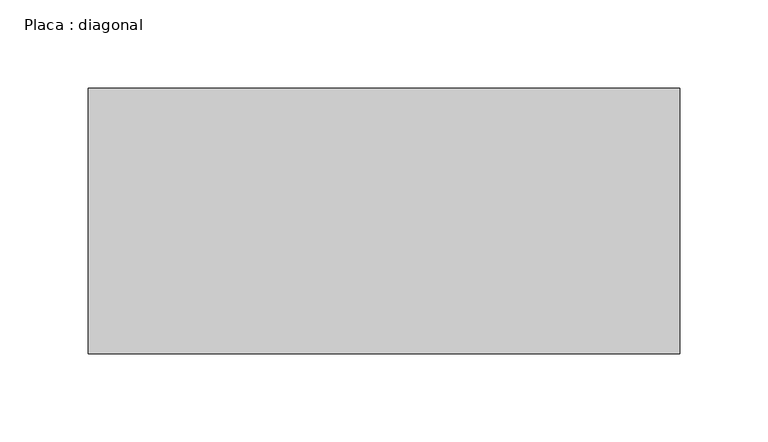
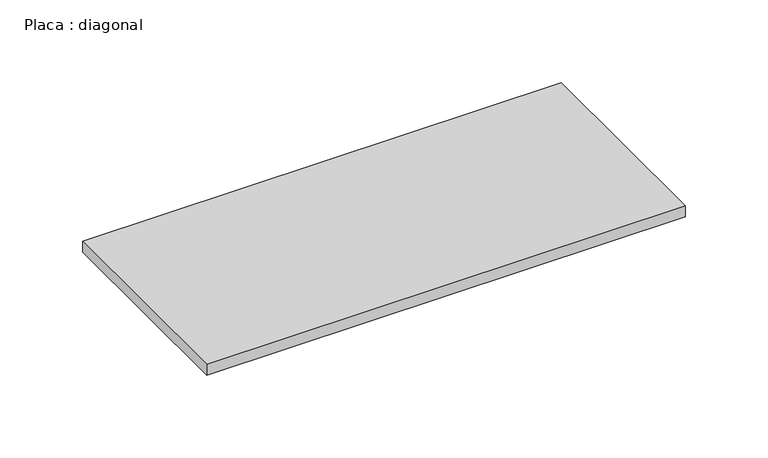
"""IFC4 building model written with IfcOpenShell, lengths in millimetres: beam geometry, Placa : diagonal."""

import ifcopenshell
import ifcopenshell.guid

model = None  # the IFC model being written
_history = None  # IfcOwnerHistory: only IFC2X3 demands one
_inside = {}  # id of a spatial element -> (the spatial element, [elements in it])
_under = {}  # id of a project, library or spatial element -> (it, [spatial elements below it])
_declared = {}  # id of a project -> (the project, [libraries it declares])
_typed = {}  # id of a type object -> (the type object, [elements of that type])
_made_of = {}  # id of a material, layer set ... -> (it, [elements and type objects made of it])


def new_model(schema):
    """Start an empty IFC model of exactly this schema.

    Asked for "IFC4X3", IfcOpenShell would pick the latest addendum, in which some entities
    have other attributes; the version numbers below select the first issue.
    IFC2X3 requires an IfcOwnerHistory on every rooted entity: one is made here for all.
    """
    global model, _history
    if schema == "IFC4X3":
        model = ifcopenshell.file(schema_version=(4, 3, 0, 0))
    else:
        model = ifcopenshell.file(schema=schema)
    _inside.clear()
    _under.clear()
    _declared.clear()
    _typed.clear()
    _made_of.clear()
    _history = None
    if model.schema == "IFC2X3":
        org = make("IfcOrganization", Name="unknown")
        user = make(
            "IfcPersonAndOrganization",
            ThePerson=make("IfcPerson", FamilyName="unknown"),
            TheOrganization=org,
        )
        app = make(
            "IfcApplication",
            ApplicationDeveloper=org,
            Version="unknown",
            ApplicationFullName="unknown",
            ApplicationIdentifier="unknown",
        )
        _history = make(
            "IfcOwnerHistory",
            OwningUser=user,
            OwningApplication=app,
            ChangeAction="ADDED",
            CreationDate=0,
        )
    return model


def make(cls, **values):
    """One entity of the class cls with the attributes given. An attribute that is None is left unset."""
    return model.create_entity(
        cls, **{name: value for name, value in values.items() if value is not None}
    )


def rooted(cls, **values):
    """An entity with a GlobalId (a new one), such as an element, a storey or a relation."""
    return make(cls, GlobalId=ifcopenshell.guid.new(), OwnerHistory=_history, **values)


def si_unit(unit_type, name, prefix=None):
    """IfcSIUnit, for example si_unit("LENGTHUNIT", "METRE", prefix="MILLI")."""
    return make("IfcSIUnit", UnitType=unit_type, Prefix=prefix, Name=name)


def assignment(units):
    """IfcUnitAssignment: the units of a project."""
    return None if units is None else make("IfcUnitAssignment", Units=units)


def point(xyz):
    """IfcCartesianPoint."""
    return None if xyz is None else make("IfcCartesianPoint", Coordinates=xyz)


def direction(xyz):
    """IfcDirection."""
    return None if xyz is None else make("IfcDirection", DirectionRatios=xyz)


def frame(location, z_axis=None, x_axis=None):
    """IfcAxis2Placement3D, a coordinate frame: its origin and axes. An axis left out is left unset."""
    return make(
        "IfcAxis2Placement3D",
        Location=point(location),
        Axis=direction(z_axis),
        RefDirection=direction(x_axis),
    )


def origin():
    """The frame at (0, 0, 0) with its axes left unset."""
    return frame((0.0, 0.0, 0.0))


def place(relative_to, where):
    """IfcLocalPlacement: puts the frame where relative to a parent placement (None: the world)."""
    return make(
        "IfcLocalPlacement", PlacementRelTo=relative_to, RelativePlacement=where
    )


def context(
    kind, dimensions, precision=None, world=None, true_north=None, identifier=None
):
    """IfcGeometricRepresentationContext, for example the 3D "Model" context."""
    return make(
        "IfcGeometricRepresentationContext",
        ContextIdentifier=identifier,
        ContextType=kind,
        CoordinateSpaceDimension=dimensions,
        Precision=precision,
        WorldCoordinateSystem=world,
        TrueNorth=true_north,
    )


def project(units=None, contexts=None):
    """IfcProject with its units and contexts."""
    return rooted(
        "IfcProject",
        Name="project",
        RepresentationContexts=contexts,
        UnitsInContext=assignment(units),
    )


def spatial(cls, under=None, at=None, **own):
    """A site, building, storey or space (cls), placed at a placement, below another one or the project."""
    s = rooted(cls, ObjectPlacement=at, **own)
    if under is not None:
        _under.setdefault(under.id(), (under, []))[1].append(s)
    return s


def polyline(points):
    """IfcPolyline through the points."""
    return make("IfcPolyline", Points=[point(p) for p in points])


def outline(outer, holes=None, kind="AREA"):
    """IfcArbitraryClosedProfileDef: a profile drawn as a closed curve; with holes, ...WithVoids."""
    if holes is None:
        return make("IfcArbitraryClosedProfileDef", ProfileType=kind, OuterCurve=outer)
    return make(
        "IfcArbitraryProfileDefWithVoids",
        ProfileType=kind,
        OuterCurve=outer,
        InnerCurves=holes,
    )


def extrude(swept, where, along, depth):
    """IfcExtrudedAreaSolid: the profile swept, set in the frame where, extruded along a direction by depth."""
    return make(
        "IfcExtrudedAreaSolid",
        SweptArea=swept,
        Position=where,
        ExtrudedDirection=direction(along),
        Depth=depth,
    )


def shape(context_of_items, identifier, shape_type, items):
    """IfcShapeRepresentation: the items that make up one representation, for example the "Body"."""
    return make(
        "IfcShapeRepresentation",
        ContextOfItems=context_of_items,
        RepresentationIdentifier=identifier,
        RepresentationType=shape_type,
        Items=items,
    )


def source(mapping_origin, context_of_items, identifier, shape_type, items):
    """IfcRepresentationMap: a shape defined once, which mapped items show again and again."""
    return make(
        "IfcRepresentationMap",
        MappingOrigin=mapping_origin,
        MappedRepresentation=shape(context_of_items, identifier, shape_type, items),
    )


def transform(
    local_origin,
    x_axis=None,
    y_axis=None,
    z_axis=None,
    scale=None,
    scale2=None,
    scale3=None,
    uniform=True,
):
    """IfcCartesianTransformationOperator3D, or its non-uniform kind. x_axis, y_axis, z_axis: its Axis1, 2, 3."""
    if uniform:
        return make(
            "IfcCartesianTransformationOperator3D",
            Axis1=direction(x_axis),
            Axis2=direction(y_axis),
            LocalOrigin=point(local_origin),
            Scale=scale,
            Axis3=direction(z_axis),
        )
    return make(
        "IfcCartesianTransformationOperator3DnonUniform",
        Axis1=direction(x_axis),
        Axis2=direction(y_axis),
        LocalOrigin=point(local_origin),
        Scale=scale,
        Axis3=direction(z_axis),
        Scale2=scale2,
        Scale3=scale3,
    )


def mapped(mapping_source, mapping_target):
    """IfcMappedItem: shows the shape of a source again, moved by a transform."""
    return make(
        "IfcMappedItem", MappingSource=mapping_source, MappingTarget=mapping_target
    )


def made_of(thing, what):
    """Note that an element or type object is made of a material, layer set ...; save() writes the relation."""
    if what is not None:
        _made_of.setdefault(what.id(), (what, []))[1].append(thing)
    return thing


def element(
    cls,
    number,
    at=None,
    inside=None,
    cuts=None,
    type_object=None,
    material=None,
    context=None,
    identifier="Body",
    shape_type=None,
    held_by="IfcProductDefinitionShape",
    body=None,
    shapes=None,
    **own,
):
    """One element of the class cls, such as IfcWall. Its Tag is "e" and its number.

    at: its placement. inside: the storey or other place that contains it. cuts: it is an
    opening in that element (IfcRelVoidsElement). A single representation is given by context,
    identifier, shape_type and body (its items); several are given by shapes. held_by: the class
    of the entity that holds the representations. save() writes the other relations.
    """
    e = rooted(cls, Tag="e%d" % number, ObjectPlacement=at, **own)
    if body is not None:
        shapes = [shape(context, identifier, shape_type, body)]
    if shapes is not None:
        e.Representation = make(held_by, Representations=shapes)
    if inside is not None:
        _inside.setdefault(inside.id(), (inside, []))[1].append(e)
    if cuts is not None:
        rooted(
            "IfcRelVoidsElement", RelatingBuildingElement=cuts, RelatedOpeningElement=e
        )
    if type_object is not None:
        _typed.setdefault(type_object.id(), (type_object, []))[1].append(e)
    return made_of(e, material)


def aggregate(whole, parts):
    """IfcRelAggregates: a whole, such as a stair, and the parts it consists of."""
    return rooted("IfcRelAggregates", RelatingObject=whole, RelatedObjects=parts)


def save(model, path):
    """Write the relations noted so far, then the file.

    IfcRelAggregates (storeys below a building ...), IfcRelContainedInSpatialStructure (elements
    in a storey), IfcRelDefinesByType, IfcRelAssociatesMaterial and IfcRelDeclares: one each for
    every whole, place, type object, material and project.
    """
    for whole, parts in _under.values():
        aggregate(whole, parts)
    for where, things in _inside.values():
        rooted(
            "IfcRelContainedInSpatialStructure",
            RelatedElements=things,
            RelatingStructure=where,
        )
    for kind, things in _typed.values():
        rooted("IfcRelDefinesByType", RelatedObjects=things, RelatingType=kind)
    for what, things in _made_of.values():
        rooted("IfcRelAssociatesMaterial", RelatedObjects=things, RelatingMaterial=what)
    for by, libraries in _declared.values():
        rooted("IfcRelDeclares", RelatingContext=by, RelatedDefinitions=libraries)
    model.write(path)


def placa_diagonal_df0326e2(model_context):
    return source(origin(), model_context, "Body", "SweptSolid", [
        extrude(outline(polyline([(167.0675395, 75.0), (167.0675395, -75.0), (-167.4240168, -75.0), (-167.4240168, 75.0), (167.0675395, 75.0)])), frame((0.0, 0.0, -4.0), z_axis=(0.0, 0.0, 1.0), x_axis=(1.0, 0.0, 0.0)), (0.0, 0.0, 1.0), 8.0),
    ])


if __name__ == "__main__":
    model = new_model("IFC4")
    model_context = context("Model", 3, world=origin())
    ifc_project = project(units=[si_unit("LENGTHUNIT", "METRE", prefix="MILLI")], contexts=[model_context])
    site = spatial("IfcSite", under=ifc_project)
    building = spatial("IfcBuilding", under=site)
    placement = place(None, origin())
    placa_diagonal_shape = placa_diagonal_df0326e2(model_context)
    element("IfcBeam", 1, ObjectType="Placa : diagonal", at=placement, inside=building, context=model_context, shape_type="MappedRepresentation", body=[
        mapped(placa_diagonal_shape, transform((0.0, 0.0, 0.0), x_axis=(1.0, 0.0, 0.0), y_axis=(0.0, 1.0, 0.0), z_axis=(0.0, 0.0, 1.0))),
    ])
    save(model, "model.ifc")

# Revit data of these elements
# Type "Placa : diagonal"
#   W = 0
#   Length [instance default] = 1.50 m
#   b = 0.15 m
#   d = 0.008 m
#   A = 0 m²
#   Structural Material [instance default] = Aço, 45-345
# Element 1 (IfcBeam, "Placa : diagonal")
#   Materials on its faces: "Aço, 45-345"
# Materials
#   "Aço, 45-345": class "Metal", colour RGB 247 247 247, transparency 0, Description = "Aço 345 MPa", Cost = 0
